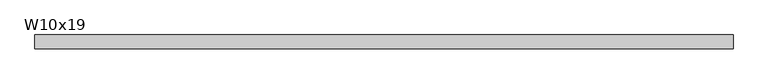
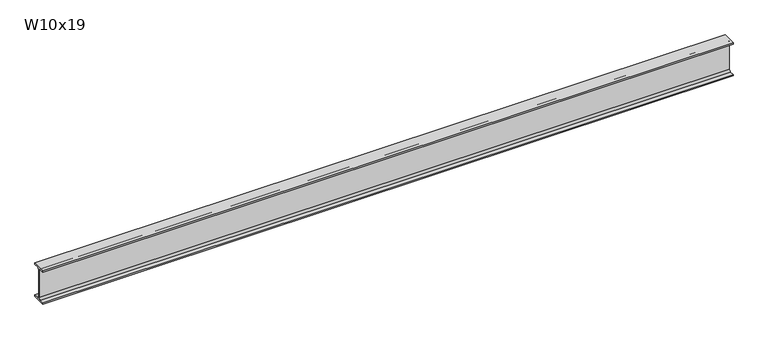
"""IFC4 building model written with IfcOpenShell, lengths in millimetres: beam geometry, RME W-Wide Flange : W10x19."""

from ifc_helpers import new_model, si_unit, point, frame, frame_2d, origin, place, context, project, spatial, polyline, circle_curve, trimmed, segment, composite_curve, outline, extrude, source, transform, mapped, element, save


def w10x19_69097861(model_context):
    return source(origin(), model_context, "Body", "SweptSolid", [
        extrude(outline(composite_curve([segment(polyline([(51.054, -119.507), (51.054, -129.54), (-51.054, -129.54), (-51.054, -119.507), (-16.9545, -119.507)]), True, "CONTINUOUS"), segment(trimmed(circle_curve(frame_2d((-16.9545, -105.7275)), 13.7795), [point((-16.9545, -119.507))], [point((-3.175, -105.7275))], True, "CARTESIAN"), True, "CONTINUOUS"), segment(polyline([(-3.175, -105.7275), (-3.175, 105.7275)]), True, "CONTINUOUS"), segment(trimmed(circle_curve(frame_2d((-16.9545, 105.7275)), 13.7795), [point((-3.175, 105.7275))], [point((-16.9545, 119.507))], True, "CARTESIAN"), True, "CONTINUOUS"), segment(polyline([(-16.9545, 119.507), (-51.054, 119.507), (-51.054, 129.54), (51.054, 129.54), (51.054, 119.507), (16.9545, 119.507)]), True, "CONTINUOUS"), segment(trimmed(circle_curve(frame_2d((16.9545, 105.7275)), 13.7795), [point((16.9545, 119.507))], [point((3.175, 105.7275))], True, "CARTESIAN"), True, "CONTINUOUS"), segment(polyline([(3.175, 105.7275), (3.175, -105.7275)]), True, "CONTINUOUS"), segment(trimmed(circle_curve(frame_2d((16.9545, -105.7275)), 13.7795), [point((3.175, -105.7275))], [point((16.9545, -119.507))], True, "CARTESIAN"), True, "CONTINUOUS"), segment(polyline([(16.9545, -119.507), (51.054, -119.507)]), True, "CONTINUOUS")], self_intersect=False)), frame((-2553.6554804, 0.0, 0.0), z_axis=(1.0, 0.0, 0.0), x_axis=(0.0, 1.0, 0.0)), (0.0, 0.0, 1.0), 5107.3109608),
    ])


if __name__ == "__main__":
    model = new_model("IFC4")
    model_context = context("Model", 3, world=origin())
    ifc_project = project(units=[si_unit("LENGTHUNIT", "METRE", prefix="MILLI")], contexts=[model_context])
    site = spatial("IfcSite", under=ifc_project)
    building = spatial("IfcBuilding", under=site)
    placement = place(None, origin())
    w10x19_shape = w10x19_69097861(model_context)
    element("IfcBeam", 1, ObjectType="RME W-Wide Flange : W10x19", at=placement, inside=building, context=model_context, shape_type="MappedRepresentation", body=[
        mapped(w10x19_shape, transform((0.0, 0.0, 0.0), x_axis=(1.0, 0.0, 0.0), y_axis=(0.0, 1.0, 0.0), z_axis=(0.0, 0.0, 1.0))),
    ])
    save(model, "model.ifc")

# Revit data of these elements
# Type "RME W-Wide Flange : W10x19"
#   WELD P [instance default] = ""
#   WELD LE [instance default] = ""
#   WELD D [instance default] = ""
#   TOP SECTION SIZE [instance default] = ""
#   TOP SECTION LENGTH [instance default] = ""
#   REMARKS [instance default] = ""
#   REINF TYPE [instance default] = ""
#   Nominal Size = "W24"
#   End Bearing Capacity [instance default] = ""
#   BOT SECTION SIZE [instance default] = ""
#   BOT SECTION LENGTH [instance default] = ""
#   Assembly Code = "B10"
#   W = 19
#   Start Extension Calculation [instance default] = 10' - 0"
#   Start Extension [instance default] = -0' - 0 1/2"
#   End Extension Calculation [instance default] = 10' - 0"
#   End Extension [instance default] = -0' - 0 1/2"
#   Length [instance default] = 5' - 0"
#   bf = 0' - 4.02"
#   d = 0' - 10.2"
#   k = 0' - 0 15/16"
#   k2 = 0' - 0.5425"
#   tf = 0' - 0.395"
#   tw = 0' - 0 1/4"
#   A = 0.0390278 SF
#   Structural Material [instance default] = Metal - Steel - ASTM A992
# Element 1 (IfcBeam, "RME W-Wide Flange : W10x19")
#   Length = 16' - 9.07523"
#   Materials on its faces: "Metal - Steel - ASTM A992"
# Materials
#   "Metal - Steel - ASTM A992": class "Metal", colour RGB 255 128 0, transparency 0
